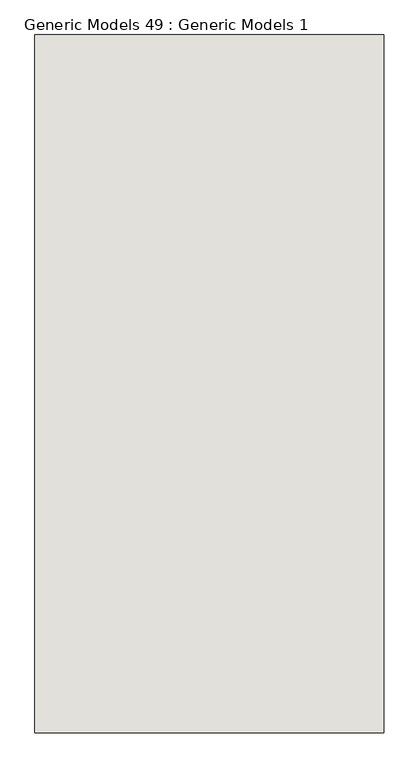
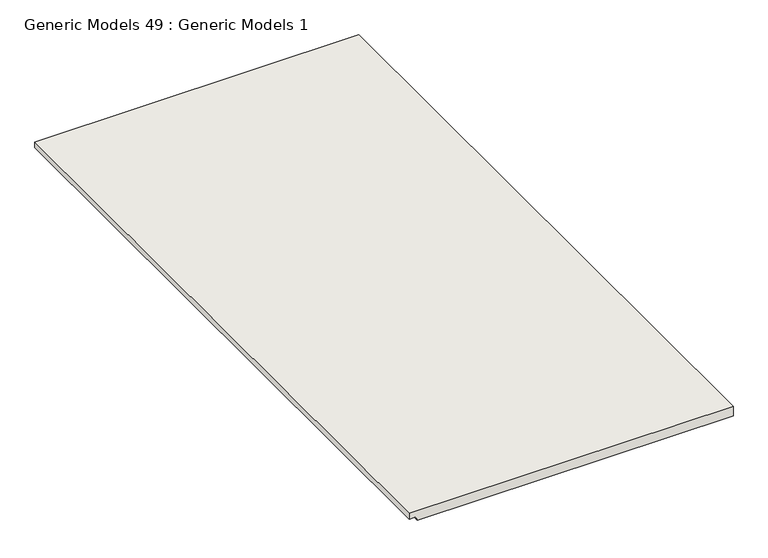
"""IFC4 building model written with IfcOpenShell, lengths in millimetres: wall geometry, Generic Models 49 : Generic Models 1."""

from ifc_helpers import new_model, si_unit, frame, origin, place, context, project, spatial, polyline, outline, extrude, source, transform, mapped, element, save


def generic_models_49_generic_models_1_cff1769b(model_context):
    return source(origin(), model_context, "Body", "SweptSolid", [
        extrude(outline(polyline([(5304.108553, 49813.3451407), (5292.996053, 49813.3451407), (5292.996053, 49826.0451407), (5285.058553, 49828.9341545), (5285.058553, 50422.9451407), (5304.108553, 50422.9451407), (5304.108553, 49813.3451407)])), frame((0.0, 0.0, 0.0), z_axis=(0.0, 1.0, 0.0), x_axis=(0.0, 0.0, 1.0)), (0.0, 0.0, 1.0), 1219.2),
    ])


if __name__ == "__main__":
    model = new_model("IFC4")
    model_context = context("Model", 3, world=origin())
    ifc_project = project(units=[si_unit("LENGTHUNIT", "METRE", prefix="MILLI")], contexts=[model_context])
    site = spatial("IfcSite", under=ifc_project)
    building = spatial("IfcBuilding", under=site)
    placement = place(None, origin())
    generic_models_49_generic_models_1_shape = generic_models_49_generic_models_1_cff1769b(model_context)
    element("IfcWall", 1, ObjectType="Generic Models 49 : Generic Models 1", at=placement, inside=building, context=model_context, shape_type="MappedRepresentation", body=[
        mapped(generic_models_49_generic_models_1_shape, transform((0.0, 0.0, 0.0), x_axis=(1.0, 0.0, 0.0), y_axis=(0.0, 1.0, 0.0), z_axis=(0.0, 0.0, 1.0))),
    ])
    save(model, "model.ifc")

# Revit data of these elements
# Element 1 (IfcWall, "Generic Models 49 : Generic Models 1")
#   Materials on its faces: "CEILING AS SCHEDULED"
# Materials
#   "CEILING AS SCHEDULED": class "Generic", colour RGB 255 255 255, transparency 0, Cost = 0
